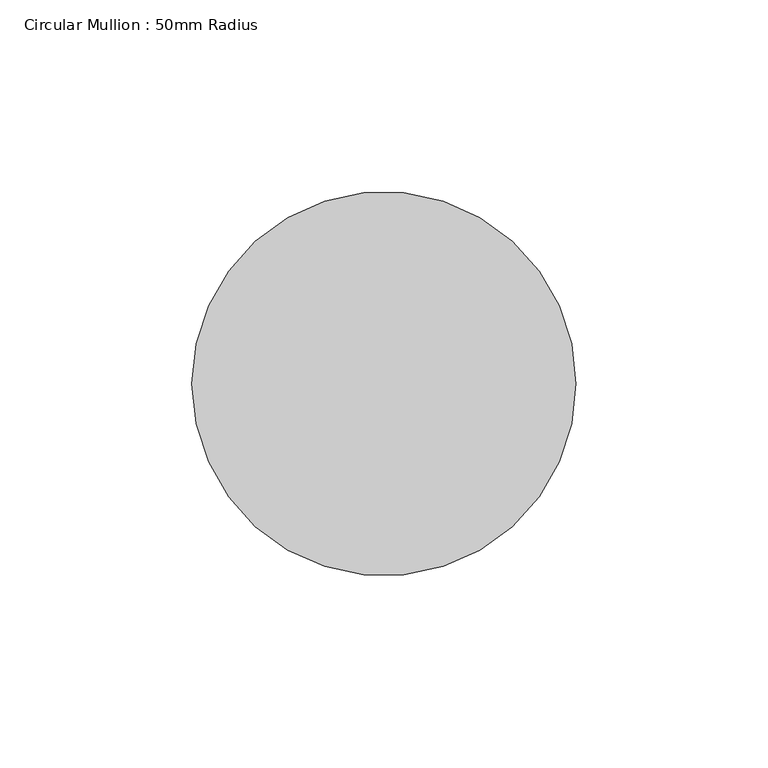
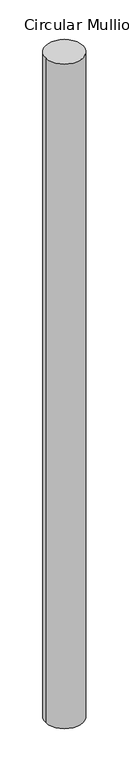
"""IFC4 building model written with IfcOpenShell, lengths in millimetres: member geometry, Circular Mullion : 50mm Radius."""

from ifc_helpers import new_model, si_unit, point, frame, frame_2d, origin, place, context, project, spatial, circle_curve, trimmed, segment, composite_curve, outline, extrude, source, transform, mapped, element, save


def circular_mullion_50mm_radius_3aeb5cb8(model_context):
    return source(origin(), model_context, "Body", "SweptSolid", [
        extrude(outline(composite_curve([segment(trimmed(circle_curve(frame_2d((-50.0, 0.0)), 50.0), [point((0.0, 0.0))], [point((-100.0, 0.0))], False, "CARTESIAN"), True, "CONTINUOUS"), segment(trimmed(circle_curve(frame_2d((-50.0, 0.0)), 50.0), [point((-100.0, 0.0))], [point((0.0, 0.0))], False, "CARTESIAN"), True, "CONTINUOUS")], self_intersect=False)), frame((0.0, 0.0, -1881.5696088), z_axis=(0.0, 0.0, 1.0), x_axis=(1.0, 0.0, 0.0)), (0.0, 0.0, 1.0), 1881.5696088),
    ])


if __name__ == "__main__":
    model = new_model("IFC4")
    model_context = context("Model", 3, world=origin())
    ifc_project = project(units=[si_unit("LENGTHUNIT", "METRE", prefix="MILLI")], contexts=[model_context])
    site = spatial("IfcSite", under=ifc_project)
    building = spatial("IfcBuilding", under=site)
    placement = place(None, origin())
    circular_mullion_50mm_radius_shape = circular_mullion_50mm_radius_3aeb5cb8(model_context)
    element("IfcMember", 1, ObjectType="Circular Mullion : 50mm Radius", at=placement, inside=building, context=model_context, shape_type="MappedRepresentation", body=[
        mapped(circular_mullion_50mm_radius_shape, transform((0.0, 0.0, 0.0), x_axis=(1.0, 0.0, 0.0), y_axis=(0.0, 1.0, 0.0), z_axis=(0.0, 0.0, 1.0))),
    ])
    save(model, "model.ifc")

# Revit data of these elements
# Type "Circular Mullion : 50mm Radius"
#   built-in parameter 1007350 = 0.164042 (stored number, unit not read)
# Element 1 (IfcMember, "Circular Mullion : 50mm Radius")
#   Materials on its faces: "Aluminium"
# Materials
#   "Aluminium": class "Metal", colour RGB 247 247 247, transparency 0, Description = "Aluminium 6061", Cost = 0
